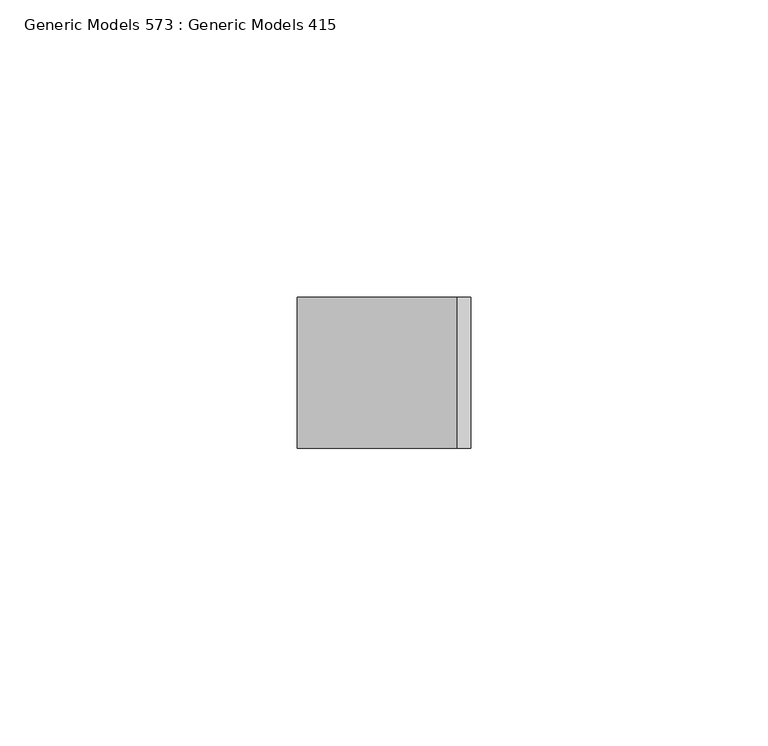
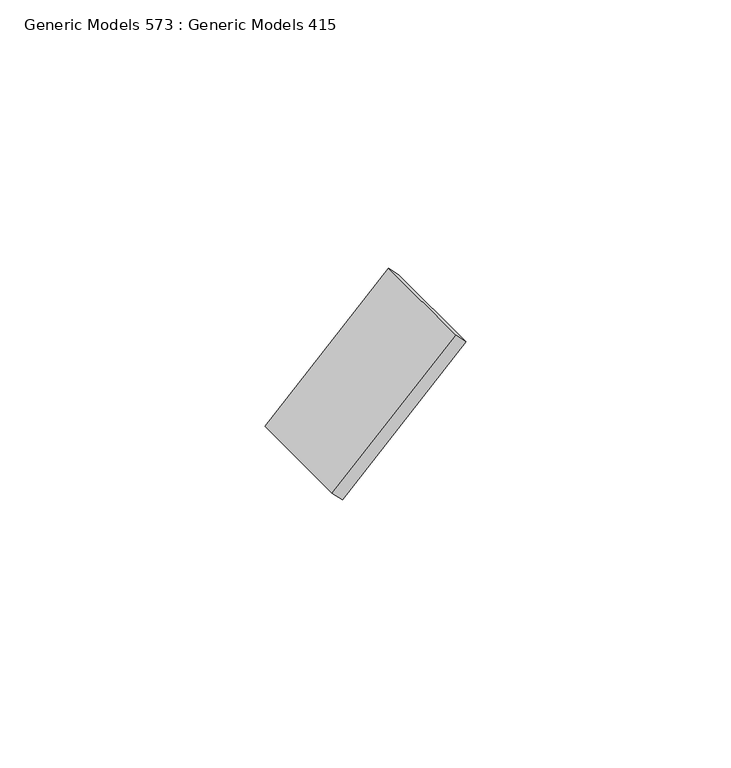
"""IFC4 building model written with IfcOpenShell, lengths in millimetres: proxy geometry, Generic Models 573 : Generic Models 415."""

from ifc_helpers import new_model, si_unit, frame, origin, place, context, project, spatial, polyline, outline, extrude, source, transform, mapped, element, save


def generic_models_573_generic_models_415_81e1f064(model_context):
    return source(origin(), model_context, "Body", "SweptSolid", [
        extrude(outline(polyline([(0.0, -3.175), (0.0, 0.0), (25.4, 0.0), (25.4, -3.175), (0.0, -3.175)])), frame((7848.0411784, 4501.3863946, 123987.8849742), z_axis=(0.7071067811867181, 0.0, 0.707106781186377), x_axis=(0.0, -1.0, 0.0)), (0.0, 0.0, 1.0), 38.1),
    ])


if __name__ == "__main__":
    model = new_model("IFC4")
    model_context = context("Model", 3, world=origin())
    ifc_project = project(units=[si_unit("LENGTHUNIT", "METRE", prefix="MILLI")], contexts=[model_context])
    site = spatial("IfcSite", under=ifc_project)
    building = spatial("IfcBuilding", under=site)
    placement = place(None, origin())
    generic_models_573_generic_models_415_shape = generic_models_573_generic_models_415_81e1f064(model_context)
    element("IfcBuildingElementProxy", 1, Name="Generic Models 573 : Generic Models 415", ObjectType="Generic Models 573 : Generic Models 415", at=placement, inside=building, context=model_context, shape_type="MappedRepresentation", body=[
        mapped(generic_models_573_generic_models_415_shape, transform((0.0, 0.0, 0.0), x_axis=(1.0, 0.0, 0.0), y_axis=(0.0, 1.0, 0.0), z_axis=(0.0, 0.0, 1.0))),
    ])
    save(model, "model.ifc")

# Revit data of these elements
# Element 1 (IfcBuildingElementProxy, "Generic Models 573 : Generic Models 415")
#   Materials on its faces: "_WELDED STEEL TABS FOR LOUVER ATTACHMENT"
# Materials
#   "_WELDED STEEL TABS FOR LOUVER ATTACHMENT": class "Metal", colour RGB 199 199 199, transparency 0, Description = "Structural steel 50ksi", Cost = 0
